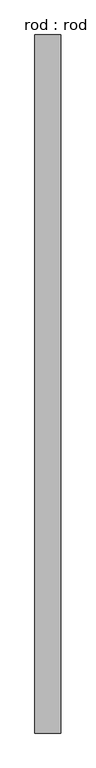
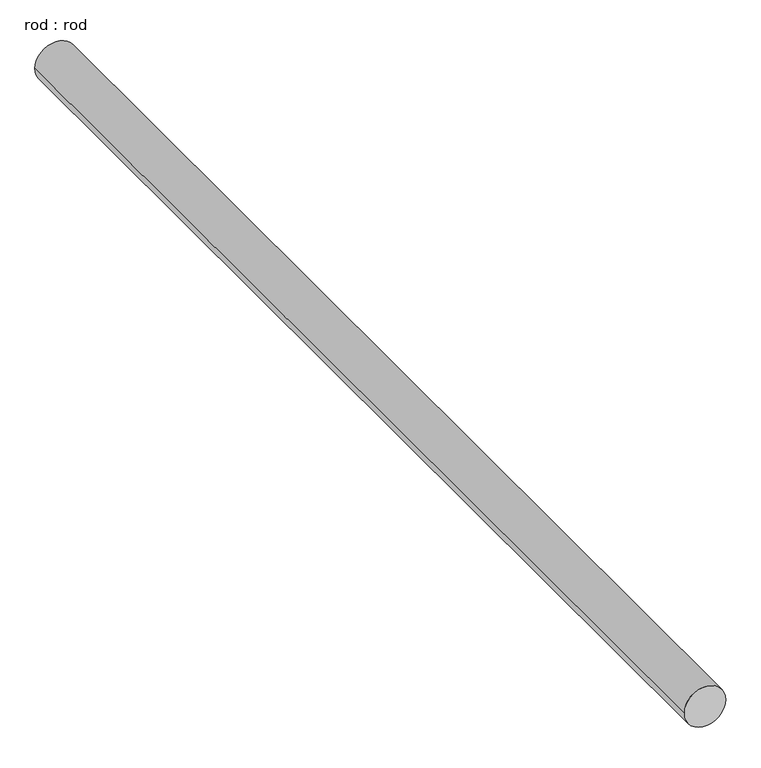
"""IFC4 building model written with IfcOpenShell, lengths in millimetres: proxy geometry, rod : rod."""

import ifcopenshell
import ifcopenshell.guid

model = None  # the IFC model being written
_history = None  # IfcOwnerHistory: only IFC2X3 demands one
_inside = {}  # id of a spatial element -> (the spatial element, [elements in it])
_under = {}  # id of a project, library or spatial element -> (it, [spatial elements below it])
_declared = {}  # id of a project -> (the project, [libraries it declares])
_typed = {}  # id of a type object -> (the type object, [elements of that type])
_made_of = {}  # id of a material, layer set ... -> (it, [elements and type objects made of it])


def new_model(schema):
    """Start an empty IFC model of exactly this schema.

    Asked for "IFC4X3", IfcOpenShell would pick the latest addendum, in which some entities
    have other attributes; the version numbers below select the first issue.
    IFC2X3 requires an IfcOwnerHistory on every rooted entity: one is made here for all.
    """
    global model, _history
    if schema == "IFC4X3":
        model = ifcopenshell.file(schema_version=(4, 3, 0, 0))
    else:
        model = ifcopenshell.file(schema=schema)
    _inside.clear()
    _under.clear()
    _declared.clear()
    _typed.clear()
    _made_of.clear()
    _history = None
    if model.schema == "IFC2X3":
        org = make("IfcOrganization", Name="unknown")
        user = make(
            "IfcPersonAndOrganization",
            ThePerson=make("IfcPerson", FamilyName="unknown"),
            TheOrganization=org,
        )
        app = make(
            "IfcApplication",
            ApplicationDeveloper=org,
            Version="unknown",
            ApplicationFullName="unknown",
            ApplicationIdentifier="unknown",
        )
        _history = make(
            "IfcOwnerHistory",
            OwningUser=user,
            OwningApplication=app,
            ChangeAction="ADDED",
            CreationDate=0,
        )
    return model


def make(cls, **values):
    """One entity of the class cls with the attributes given. An attribute that is None is left unset."""
    return model.create_entity(
        cls, **{name: value for name, value in values.items() if value is not None}
    )


def rooted(cls, **values):
    """An entity with a GlobalId (a new one), such as an element, a storey or a relation."""
    return make(cls, GlobalId=ifcopenshell.guid.new(), OwnerHistory=_history, **values)


def si_unit(unit_type, name, prefix=None):
    """IfcSIUnit, for example si_unit("LENGTHUNIT", "METRE", prefix="MILLI")."""
    return make("IfcSIUnit", UnitType=unit_type, Prefix=prefix, Name=name)


def assignment(units):
    """IfcUnitAssignment: the units of a project."""
    return None if units is None else make("IfcUnitAssignment", Units=units)


def point(xyz):
    """IfcCartesianPoint."""
    return None if xyz is None else make("IfcCartesianPoint", Coordinates=xyz)


def direction(xyz):
    """IfcDirection."""
    return None if xyz is None else make("IfcDirection", DirectionRatios=xyz)


def frame(location, z_axis=None, x_axis=None):
    """IfcAxis2Placement3D, a coordinate frame: its origin and axes. An axis left out is left unset."""
    return make(
        "IfcAxis2Placement3D",
        Location=point(location),
        Axis=direction(z_axis),
        RefDirection=direction(x_axis),
    )


def frame_2d(location, x_axis=None):
    """IfcAxis2Placement2D, a coordinate frame in the plane: its origin and x axis."""
    return make(
        "IfcAxis2Placement2D", Location=point(location), RefDirection=direction(x_axis)
    )


def origin():
    """The frame at (0, 0, 0) with its axes left unset."""
    return frame((0.0, 0.0, 0.0))


def place(relative_to, where):
    """IfcLocalPlacement: puts the frame where relative to a parent placement (None: the world)."""
    return make(
        "IfcLocalPlacement", PlacementRelTo=relative_to, RelativePlacement=where
    )


def context(
    kind, dimensions, precision=None, world=None, true_north=None, identifier=None
):
    """IfcGeometricRepresentationContext, for example the 3D "Model" context."""
    return make(
        "IfcGeometricRepresentationContext",
        ContextIdentifier=identifier,
        ContextType=kind,
        CoordinateSpaceDimension=dimensions,
        Precision=precision,
        WorldCoordinateSystem=world,
        TrueNorth=true_north,
    )


def project(units=None, contexts=None):
    """IfcProject with its units and contexts."""
    return rooted(
        "IfcProject",
        Name="project",
        RepresentationContexts=contexts,
        UnitsInContext=assignment(units),
    )


def spatial(cls, under=None, at=None, **own):
    """A site, building, storey or space (cls), placed at a placement, below another one or the project."""
    s = rooted(cls, ObjectPlacement=at, **own)
    if under is not None:
        _under.setdefault(under.id(), (under, []))[1].append(s)
    return s


def circle_curve(where, radius):
    """IfcCircle in the frame where."""
    return make("IfcCircle", Position=where, Radius=radius)


def trimmed(basis, trim1, trim2, sense, master):
    """IfcTrimmedCurve: the piece of a basis curve between two trims."""
    return make(
        "IfcTrimmedCurve",
        BasisCurve=basis,
        Trim1=trim1,
        Trim2=trim2,
        SenseAgreement=sense,
        MasterRepresentation=master,
    )


def segment(curve, same_sense, transition):
    """IfcCompositeCurveSegment."""
    return make(
        "IfcCompositeCurveSegment",
        Transition=transition,
        SameSense=same_sense,
        ParentCurve=curve,
    )


def composite_curve(segments, self_intersect=None):
    """IfcCompositeCurve: segments joined end to end."""
    return make("IfcCompositeCurve", Segments=segments, SelfIntersect=self_intersect)


def outline(outer, holes=None, kind="AREA"):
    """IfcArbitraryClosedProfileDef: a profile drawn as a closed curve; with holes, ...WithVoids."""
    if holes is None:
        return make("IfcArbitraryClosedProfileDef", ProfileType=kind, OuterCurve=outer)
    return make(
        "IfcArbitraryProfileDefWithVoids",
        ProfileType=kind,
        OuterCurve=outer,
        InnerCurves=holes,
    )


def extrude(swept, where, along, depth):
    """IfcExtrudedAreaSolid: the profile swept, set in the frame where, extruded along a direction by depth."""
    return make(
        "IfcExtrudedAreaSolid",
        SweptArea=swept,
        Position=where,
        ExtrudedDirection=direction(along),
        Depth=depth,
    )


def shape(context_of_items, identifier, shape_type, items):
    """IfcShapeRepresentation: the items that make up one representation, for example the "Body"."""
    return make(
        "IfcShapeRepresentation",
        ContextOfItems=context_of_items,
        RepresentationIdentifier=identifier,
        RepresentationType=shape_type,
        Items=items,
    )


def source(mapping_origin, context_of_items, identifier, shape_type, items):
    """IfcRepresentationMap: a shape defined once, which mapped items show again and again."""
    return make(
        "IfcRepresentationMap",
        MappingOrigin=mapping_origin,
        MappedRepresentation=shape(context_of_items, identifier, shape_type, items),
    )


def transform(
    local_origin,
    x_axis=None,
    y_axis=None,
    z_axis=None,
    scale=None,
    scale2=None,
    scale3=None,
    uniform=True,
):
    """IfcCartesianTransformationOperator3D, or its non-uniform kind. x_axis, y_axis, z_axis: its Axis1, 2, 3."""
    if uniform:
        return make(
            "IfcCartesianTransformationOperator3D",
            Axis1=direction(x_axis),
            Axis2=direction(y_axis),
            LocalOrigin=point(local_origin),
            Scale=scale,
            Axis3=direction(z_axis),
        )
    return make(
        "IfcCartesianTransformationOperator3DnonUniform",
        Axis1=direction(x_axis),
        Axis2=direction(y_axis),
        LocalOrigin=point(local_origin),
        Scale=scale,
        Axis3=direction(z_axis),
        Scale2=scale2,
        Scale3=scale3,
    )


def mapped(mapping_source, mapping_target):
    """IfcMappedItem: shows the shape of a source again, moved by a transform."""
    return make(
        "IfcMappedItem", MappingSource=mapping_source, MappingTarget=mapping_target
    )


def made_of(thing, what):
    """Note that an element or type object is made of a material, layer set ...; save() writes the relation."""
    if what is not None:
        _made_of.setdefault(what.id(), (what, []))[1].append(thing)
    return thing


def element(
    cls,
    number,
    at=None,
    inside=None,
    cuts=None,
    type_object=None,
    material=None,
    context=None,
    identifier="Body",
    shape_type=None,
    held_by="IfcProductDefinitionShape",
    body=None,
    shapes=None,
    **own,
):
    """One element of the class cls, such as IfcWall. Its Tag is "e" and its number.

    at: its placement. inside: the storey or other place that contains it. cuts: it is an
    opening in that element (IfcRelVoidsElement). A single representation is given by context,
    identifier, shape_type and body (its items); several are given by shapes. held_by: the class
    of the entity that holds the representations. save() writes the other relations.
    """
    e = rooted(cls, Tag="e%d" % number, ObjectPlacement=at, **own)
    if body is not None:
        shapes = [shape(context, identifier, shape_type, body)]
    if shapes is not None:
        e.Representation = make(held_by, Representations=shapes)
    if inside is not None:
        _inside.setdefault(inside.id(), (inside, []))[1].append(e)
    if cuts is not None:
        rooted(
            "IfcRelVoidsElement", RelatingBuildingElement=cuts, RelatedOpeningElement=e
        )
    if type_object is not None:
        _typed.setdefault(type_object.id(), (type_object, []))[1].append(e)
    return made_of(e, material)


def aggregate(whole, parts):
    """IfcRelAggregates: a whole, such as a stair, and the parts it consists of."""
    return rooted("IfcRelAggregates", RelatingObject=whole, RelatedObjects=parts)


def save(model, path):
    """Write the relations noted so far, then the file.

    IfcRelAggregates (storeys below a building ...), IfcRelContainedInSpatialStructure (elements
    in a storey), IfcRelDefinesByType, IfcRelAssociatesMaterial and IfcRelDeclares: one each for
    every whole, place, type object, material and project.
    """
    for whole, parts in _under.values():
        aggregate(whole, parts)
    for where, things in _inside.values():
        rooted(
            "IfcRelContainedInSpatialStructure",
            RelatedElements=things,
            RelatingStructure=where,
        )
    for kind, things in _typed.values():
        rooted("IfcRelDefinesByType", RelatedObjects=things, RelatingType=kind)
    for what, things in _made_of.values():
        rooted("IfcRelAssociatesMaterial", RelatedObjects=things, RelatingMaterial=what)
    for by, libraries in _declared.values():
        rooted("IfcRelDeclares", RelatingContext=by, RelatedDefinitions=libraries)
    model.write(path)


def rod_rod_bee4bf64(model_context):
    return source(origin(), model_context, "Body", "SweptSolid", [
        extrude(outline(composite_curve([segment(trimmed(circle_curve(frame_2d((0.0108462, 0.0)), 200.0), [point((0.0108462, 200.0))], [point((0.0108462, -200.0))], False, "CARTESIAN"), True, "CONTINUOUS"), segment(trimmed(circle_curve(frame_2d((0.0108462, 0.0)), 200.0), [point((0.0108462, -200.0))], [point((0.0108462, 200.0))], False, "CARTESIAN"), True, "CONTINUOUS")], self_intersect=False)), frame((0.0, -1300.1285275, 0.0), z_axis=(0.0, 1.0, 0.0), x_axis=(0.0, 0.0, 1.0)), (0.0, 0.0, 1.0), 10785.7142857),
    ])


if __name__ == "__main__":
    model = new_model("IFC4")
    model_context = context("Model", 3, world=origin())
    ifc_project = project(units=[si_unit("LENGTHUNIT", "METRE", prefix="MILLI")], contexts=[model_context])
    site = spatial("IfcSite", under=ifc_project)
    building = spatial("IfcBuilding", under=site)
    placement = place(None, origin())
    rod_rod_shape = rod_rod_bee4bf64(model_context)
    element("IfcBuildingElementProxy", 1, Name="rod : rod", ObjectType="rod : rod", at=placement, inside=building, context=model_context, shape_type="MappedRepresentation", body=[
        mapped(rod_rod_shape, transform((0.0, 0.0, 0.0), x_axis=(1.0, 0.0, 0.0), y_axis=(0.0, 1.0, 0.0), z_axis=(0.0, 0.0, 1.0))),
    ])
    save(model, "model.ifc")

# Revit data of these elements
# Type "rod : rod"
#   Default Elevation = 0
